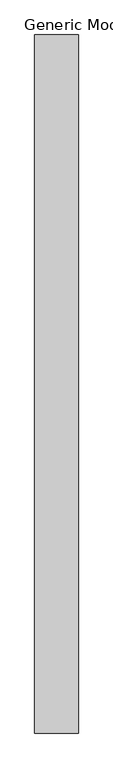
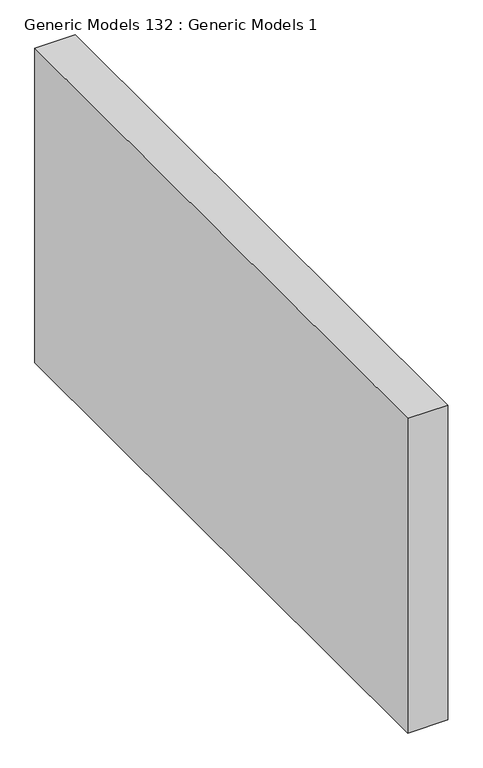
"""IFC4 building model written with IfcOpenShell, lengths in millimetres: proxy geometry, Generic Models 132 : Generic Models 1."""

from ifc_helpers import new_model, si_unit, frame, origin, place, context, project, spatial, polyline, outline, extrude, source, transform, mapped, element, save


def generic_models_132_generic_models_1_954f0ab9(model_context):
    return source(origin(), model_context, "Body", "SweptSolid", [
        extrude(outline(polyline([(48147.1360531, 1219.2), (48147.1360531, 0.0), (48070.9360531, 0.0), (48070.9360531, 1219.2), (48147.1360531, 1219.2)])), frame((0.0, 0.0, 1598.2598705), z_axis=(0.0, 0.0, 1.0), x_axis=(1.0, 0.0, 0.0)), (0.0, 0.0, 1.0), 628.4515625),
    ])


if __name__ == "__main__":
    model = new_model("IFC4")
    model_context = context("Model", 3, world=origin())
    ifc_project = project(units=[si_unit("LENGTHUNIT", "METRE", prefix="MILLI")], contexts=[model_context])
    site = spatial("IfcSite", under=ifc_project)
    building = spatial("IfcBuilding", under=site)
    placement = place(None, origin())
    generic_models_132_generic_models_1_shape = generic_models_132_generic_models_1_954f0ab9(model_context)
    element("IfcBuildingElementProxy", 1, Name="Generic Models 132 : Generic Models 1", ObjectType="Generic Models 132 : Generic Models 1", at=placement, inside=building, context=model_context, shape_type="MappedRepresentation", body=[
        mapped(generic_models_132_generic_models_1_shape, transform((0.0, 0.0, 0.0), x_axis=(1.0, 0.0, 0.0), y_axis=(0.0, 1.0, 0.0), z_axis=(0.0, 0.0, 1.0))),
    ])
    save(model, "model.ifc")

# Revit data of these elements
# Element 1 (IfcBuildingElementProxy, "Generic Models 132 : Generic Models 1")
#   Materials on its faces: "(S) SOUND BATT. INSULATION (THICKNESS TO MATCH WALL DEPTH)"
# Materials
#   "(S) SOUND BATT. INSULATION (THICKNESS TO MATCH WALL DEPTH)": class "Unassigned", colour RGB 255 255 255, transparency 0, Cost = 0
